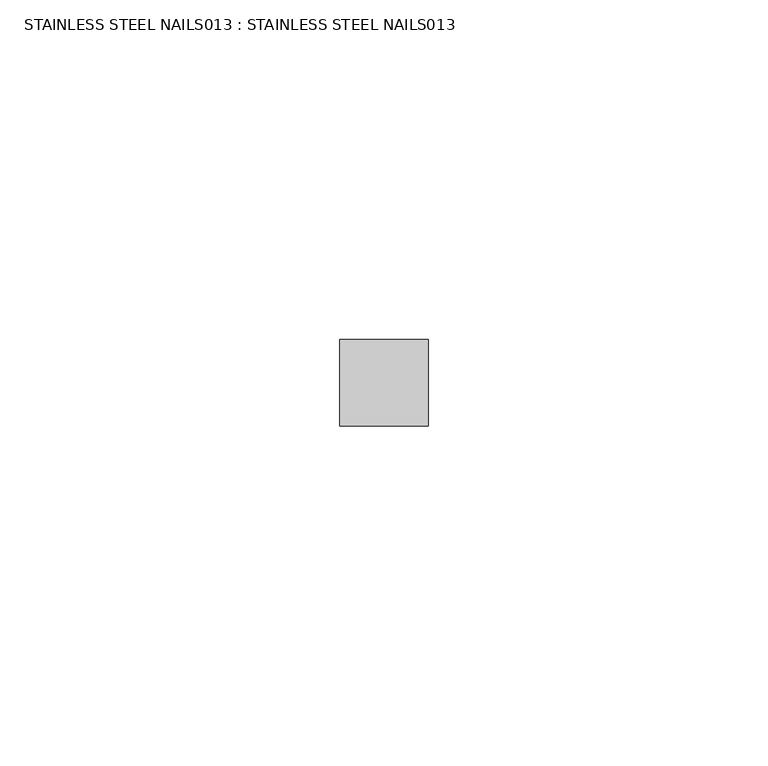
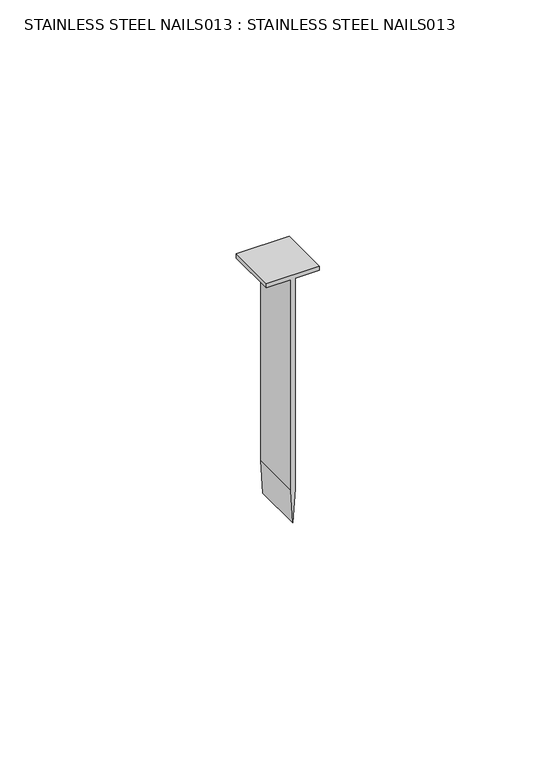
"""IFC4 building model written with IfcOpenShell, lengths in millimetres: proxy geometry, STAINLESS STEEL NAILS013 : STAINLESS STEEL NAILS013."""

import ifcopenshell
import ifcopenshell.guid

model = None  # the IFC model being written
_history = None  # IfcOwnerHistory: only IFC2X3 demands one
_inside = {}  # id of a spatial element -> (the spatial element, [elements in it])
_under = {}  # id of a project, library or spatial element -> (it, [spatial elements below it])
_declared = {}  # id of a project -> (the project, [libraries it declares])
_typed = {}  # id of a type object -> (the type object, [elements of that type])
_made_of = {}  # id of a material, layer set ... -> (it, [elements and type objects made of it])


def new_model(schema):
    """Start an empty IFC model of exactly this schema.

    Asked for "IFC4X3", IfcOpenShell would pick the latest addendum, in which some entities
    have other attributes; the version numbers below select the first issue.
    IFC2X3 requires an IfcOwnerHistory on every rooted entity: one is made here for all.
    """
    global model, _history
    if schema == "IFC4X3":
        model = ifcopenshell.file(schema_version=(4, 3, 0, 0))
    else:
        model = ifcopenshell.file(schema=schema)
    _inside.clear()
    _under.clear()
    _declared.clear()
    _typed.clear()
    _made_of.clear()
    _history = None
    if model.schema == "IFC2X3":
        org = make("IfcOrganization", Name="unknown")
        user = make(
            "IfcPersonAndOrganization",
            ThePerson=make("IfcPerson", FamilyName="unknown"),
            TheOrganization=org,
        )
        app = make(
            "IfcApplication",
            ApplicationDeveloper=org,
            Version="unknown",
            ApplicationFullName="unknown",
            ApplicationIdentifier="unknown",
        )
        _history = make(
            "IfcOwnerHistory",
            OwningUser=user,
            OwningApplication=app,
            ChangeAction="ADDED",
            CreationDate=0,
        )
    return model


def make(cls, **values):
    """One entity of the class cls with the attributes given. An attribute that is None is left unset."""
    return model.create_entity(
        cls, **{name: value for name, value in values.items() if value is not None}
    )


def rooted(cls, **values):
    """An entity with a GlobalId (a new one), such as an element, a storey or a relation."""
    return make(cls, GlobalId=ifcopenshell.guid.new(), OwnerHistory=_history, **values)


def si_unit(unit_type, name, prefix=None):
    """IfcSIUnit, for example si_unit("LENGTHUNIT", "METRE", prefix="MILLI")."""
    return make("IfcSIUnit", UnitType=unit_type, Prefix=prefix, Name=name)


def assignment(units):
    """IfcUnitAssignment: the units of a project."""
    return None if units is None else make("IfcUnitAssignment", Units=units)


def point(xyz):
    """IfcCartesianPoint."""
    return None if xyz is None else make("IfcCartesianPoint", Coordinates=xyz)


def direction(xyz):
    """IfcDirection."""
    return None if xyz is None else make("IfcDirection", DirectionRatios=xyz)


def frame(location, z_axis=None, x_axis=None):
    """IfcAxis2Placement3D, a coordinate frame: its origin and axes. An axis left out is left unset."""
    return make(
        "IfcAxis2Placement3D",
        Location=point(location),
        Axis=direction(z_axis),
        RefDirection=direction(x_axis),
    )


def origin():
    """The frame at (0, 0, 0) with its axes left unset."""
    return frame((0.0, 0.0, 0.0))


def place(relative_to, where):
    """IfcLocalPlacement: puts the frame where relative to a parent placement (None: the world)."""
    return make(
        "IfcLocalPlacement", PlacementRelTo=relative_to, RelativePlacement=where
    )


def context(
    kind, dimensions, precision=None, world=None, true_north=None, identifier=None
):
    """IfcGeometricRepresentationContext, for example the 3D "Model" context."""
    return make(
        "IfcGeometricRepresentationContext",
        ContextIdentifier=identifier,
        ContextType=kind,
        CoordinateSpaceDimension=dimensions,
        Precision=precision,
        WorldCoordinateSystem=world,
        TrueNorth=true_north,
    )


def project(units=None, contexts=None):
    """IfcProject with its units and contexts."""
    return rooted(
        "IfcProject",
        Name="project",
        RepresentationContexts=contexts,
        UnitsInContext=assignment(units),
    )


def spatial(cls, under=None, at=None, **own):
    """A site, building, storey or space (cls), placed at a placement, below another one or the project."""
    s = rooted(cls, ObjectPlacement=at, **own)
    if under is not None:
        _under.setdefault(under.id(), (under, []))[1].append(s)
    return s


def polyline(points):
    """IfcPolyline through the points."""
    return make("IfcPolyline", Points=[point(p) for p in points])


def outline(outer, holes=None, kind="AREA"):
    """IfcArbitraryClosedProfileDef: a profile drawn as a closed curve; with holes, ...WithVoids."""
    if holes is None:
        return make("IfcArbitraryClosedProfileDef", ProfileType=kind, OuterCurve=outer)
    return make(
        "IfcArbitraryProfileDefWithVoids",
        ProfileType=kind,
        OuterCurve=outer,
        InnerCurves=holes,
    )


def extrude(swept, where, along, depth):
    """IfcExtrudedAreaSolid: the profile swept, set in the frame where, extruded along a direction by depth."""
    return make(
        "IfcExtrudedAreaSolid",
        SweptArea=swept,
        Position=where,
        ExtrudedDirection=direction(along),
        Depth=depth,
    )


def shape(context_of_items, identifier, shape_type, items):
    """IfcShapeRepresentation: the items that make up one representation, for example the "Body"."""
    return make(
        "IfcShapeRepresentation",
        ContextOfItems=context_of_items,
        RepresentationIdentifier=identifier,
        RepresentationType=shape_type,
        Items=items,
    )


def source(mapping_origin, context_of_items, identifier, shape_type, items):
    """IfcRepresentationMap: a shape defined once, which mapped items show again and again."""
    return make(
        "IfcRepresentationMap",
        MappingOrigin=mapping_origin,
        MappedRepresentation=shape(context_of_items, identifier, shape_type, items),
    )


def transform(
    local_origin,
    x_axis=None,
    y_axis=None,
    z_axis=None,
    scale=None,
    scale2=None,
    scale3=None,
    uniform=True,
):
    """IfcCartesianTransformationOperator3D, or its non-uniform kind. x_axis, y_axis, z_axis: its Axis1, 2, 3."""
    if uniform:
        return make(
            "IfcCartesianTransformationOperator3D",
            Axis1=direction(x_axis),
            Axis2=direction(y_axis),
            LocalOrigin=point(local_origin),
            Scale=scale,
            Axis3=direction(z_axis),
        )
    return make(
        "IfcCartesianTransformationOperator3DnonUniform",
        Axis1=direction(x_axis),
        Axis2=direction(y_axis),
        LocalOrigin=point(local_origin),
        Scale=scale,
        Axis3=direction(z_axis),
        Scale2=scale2,
        Scale3=scale3,
    )


def mapped(mapping_source, mapping_target):
    """IfcMappedItem: shows the shape of a source again, moved by a transform."""
    return make(
        "IfcMappedItem", MappingSource=mapping_source, MappingTarget=mapping_target
    )


def made_of(thing, what):
    """Note that an element or type object is made of a material, layer set ...; save() writes the relation."""
    if what is not None:
        _made_of.setdefault(what.id(), (what, []))[1].append(thing)
    return thing


def element(
    cls,
    number,
    at=None,
    inside=None,
    cuts=None,
    type_object=None,
    material=None,
    context=None,
    identifier="Body",
    shape_type=None,
    held_by="IfcProductDefinitionShape",
    body=None,
    shapes=None,
    **own,
):
    """One element of the class cls, such as IfcWall. Its Tag is "e" and its number.

    at: its placement. inside: the storey or other place that contains it. cuts: it is an
    opening in that element (IfcRelVoidsElement). A single representation is given by context,
    identifier, shape_type and body (its items); several are given by shapes. held_by: the class
    of the entity that holds the representations. save() writes the other relations.
    """
    e = rooted(cls, Tag="e%d" % number, ObjectPlacement=at, **own)
    if body is not None:
        shapes = [shape(context, identifier, shape_type, body)]
    if shapes is not None:
        e.Representation = make(held_by, Representations=shapes)
    if inside is not None:
        _inside.setdefault(inside.id(), (inside, []))[1].append(e)
    if cuts is not None:
        rooted(
            "IfcRelVoidsElement", RelatingBuildingElement=cuts, RelatedOpeningElement=e
        )
    if type_object is not None:
        _typed.setdefault(type_object.id(), (type_object, []))[1].append(e)
    return made_of(e, material)


def aggregate(whole, parts):
    """IfcRelAggregates: a whole, such as a stair, and the parts it consists of."""
    return rooted("IfcRelAggregates", RelatingObject=whole, RelatedObjects=parts)


def save(model, path):
    """Write the relations noted so far, then the file.

    IfcRelAggregates (storeys below a building ...), IfcRelContainedInSpatialStructure (elements
    in a storey), IfcRelDefinesByType, IfcRelAssociatesMaterial and IfcRelDeclares: one each for
    every whole, place, type object, material and project.
    """
    for whole, parts in _under.values():
        aggregate(whole, parts)
    for where, things in _inside.values():
        rooted(
            "IfcRelContainedInSpatialStructure",
            RelatedElements=things,
            RelatingStructure=where,
        )
    for kind, things in _typed.values():
        rooted("IfcRelDefinesByType", RelatedObjects=things, RelatingType=kind)
    for what, things in _made_of.values():
        rooted("IfcRelAssociatesMaterial", RelatedObjects=things, RelatingMaterial=what)
    for by, libraries in _declared.values():
        rooted("IfcRelDeclares", RelatingContext=by, RelatedDefinitions=libraries)
    model.write(path)


def stainless_steel_nails013_stainless_steel_nails013_b095092e(model_context):
    return source(origin(), model_context, "Body", "SweptSolid", [
        extrude(outline(polyline([(40259.5998489, -4931.7136341), (40259.5998489, -4925.7560415), (40205.2729558, -4925.7560415), (40196.6073666, -4925.2144421), (40205.2729558, -4924.6728428), (40259.5998489, -4924.6728428), (40259.5998489, -4918.7152502), (40260.6830476, -4918.7152502), (40260.6830476, -4931.7136341), (40259.5998489, -4931.7136341)])), frame((0.0, -1065.5906573, 0.0), z_axis=(0.0, 1.0, 0.0), x_axis=(0.0, 0.0, 1.0)), (0.0, 0.0, 1.0), 12.7),
    ])


if __name__ == "__main__":
    model = new_model("IFC4")
    model_context = context("Model", 3, world=origin())
    ifc_project = project(units=[si_unit("LENGTHUNIT", "METRE", prefix="MILLI")], contexts=[model_context])
    site = spatial("IfcSite", under=ifc_project)
    building = spatial("IfcBuilding", under=site)
    placement = place(None, origin())
    stainless_steel_nails013_stainless_steel_nails013_shape = stainless_steel_nails013_stainless_steel_nails013_b095092e(model_context)
    element("IfcBuildingElementProxy", 1, Name="STAINLESS STEEL NAILS013 : STAINLESS STEEL NAILS013", ObjectType="STAINLESS STEEL NAILS013 : STAINLESS STEEL NAILS013", at=placement, inside=building, context=model_context, shape_type="MappedRepresentation", body=[
        mapped(stainless_steel_nails013_stainless_steel_nails013_shape, transform((0.0, 0.0, 0.0), x_axis=(1.0, 0.0, 0.0), y_axis=(0.0, 1.0, 0.0), z_axis=(0.0, 0.0, 1.0))),
    ])
    save(model, "model.ifc")

# Revit data of these elements
# Type "STAINLESS STEEL NAILS013 : STAINLESS STEEL NAILS013"
#   NameOverride = "STAINLESS STEEL NAILS013"
# Element 1 (IfcBuildingElementProxy, "STAINLESS STEEL NAILS013 : STAINLESS STEEL NAILS013")
#   Materials on its faces: "1 3/4\" STAINLESS STEEL RINGSHANK 5D COMMON NAILS @ 4\" (101.6MM) O.C. FIRESTONE PROVIDED MAX., 1/2\" STAGGERED"
# Materials
#   "1 3/4\" STAINLESS STEEL RINGSHANK 5D COMMON NAILS @ 4\" (101.6MM) O.C. FIRESTONE PROVIDED MAX., 1/2\" STAGGERED": class "Unassigned", colour RGB 255 255 255, transparency 0
